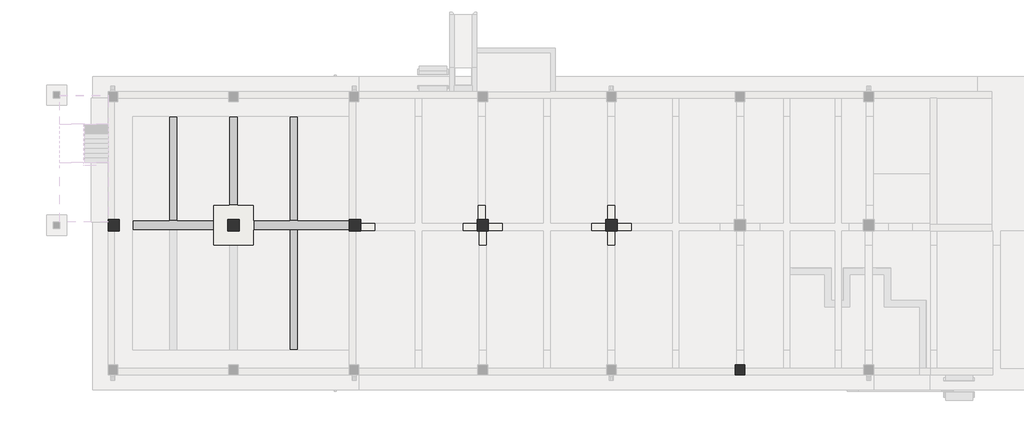
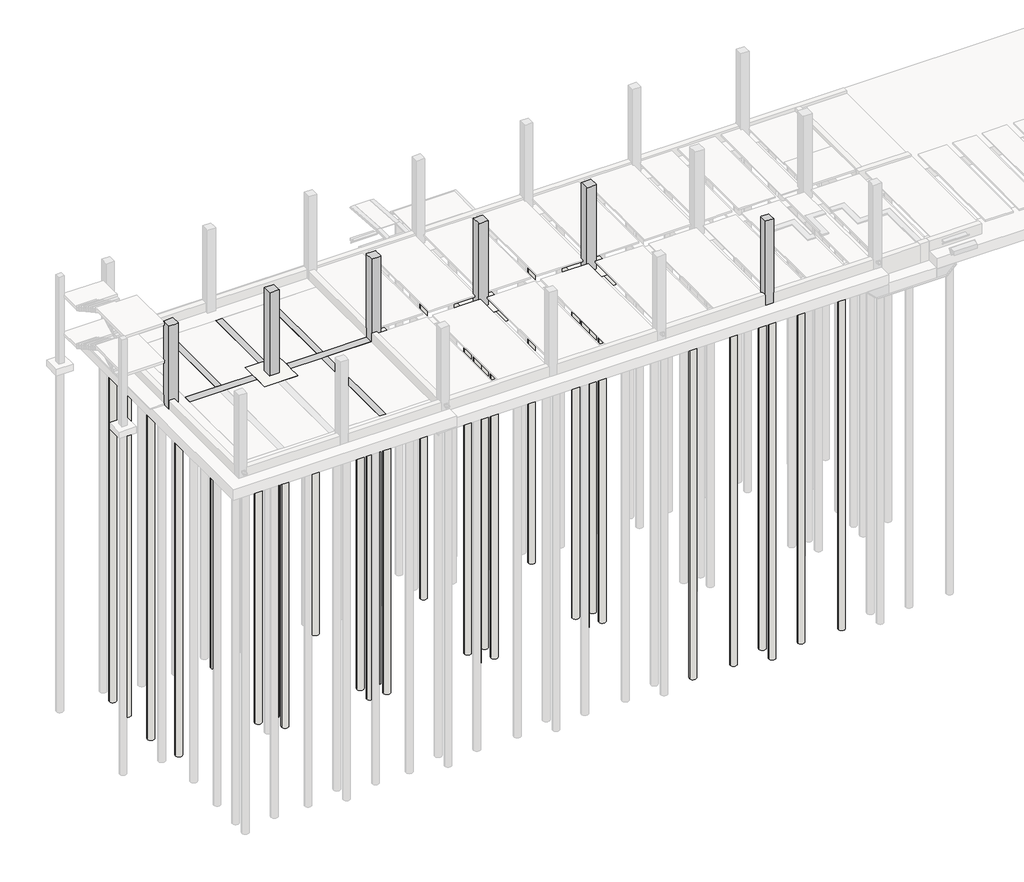
# One storey, part 4 of 7: 33 slabs, 8 beams, 6 columns.
"""IFC4 building model written with IfcOpenShell, lengths in millimetres."""

from ifc_helpers import new_model, si_unit, point, frame, frame_2d, origin, place, context, project, spatial, polyline, circle_curve, trimmed, segment, composite_curve, outline, extrude, faceted_brep, element, save

model = new_model("IFC4")

# Units and contexts
model_context = context("Model", 3, world=origin())
ifc_project = project(units=[si_unit("LENGTHUNIT", "METRE", prefix="MILLI")], contexts=[model_context])

# Site, building, storey
site = spatial("IfcSite", under=ifc_project)
building = spatial("IfcBuilding", under=site)
storey = spatial("IfcBuildingStorey", under=building, Name="H.P.P", Elevation=4500.0)

# Beams
placement = place(None, origin())
element("IfcBeam", 1, ObjectType="RC Beam_Rectangular : H_SB_AR S16_TG-UG_500x700_FB1A", at=placement, inside=storey, context=model_context, shape_type="Brep", body=[
    faceted_brep([(11000.0, -15750.0, 3400.0), (11500.0, -15750.0, 3400.0), (11500.0, -15750.0, 3840.0), (11500.0, -15750.0, 3950.0), (11500.0, -15750.0, 4100.0), (11000.0, -15750.0, 4100.0), (11000.0, -15750.0, 3950.0), (11000.0, -15750.0, 3840.0), (11500.0, -8299.9999999, 4100.0), (11000.0, -8299.9999999, 4100.0), (11500.0, -8299.9999999, 3950.0), (11500.0, -8299.9999999, 3400.0), (11500.0, -8299.9999999, 3840.0), (11000.0, -8299.9999999, 3400.0), (11000.0, -8299.9999999, 3950.0), (11000.0, -8299.9999999, 3840.0)], [[[0, 1, 2, 3, 4, 5, 6, 7]], [[5, 4, 8, 9]], [[10, 8, 4, 3, 2, 1, 11, 12]], [[1, 0, 13, 11]], [[9, 14, 15, 13, 0, 7, 6, 5]], [[9, 8, 10, 12, 11, 13, 15, 14]]]),
])
element("IfcBeam", 2, ObjectType="RC Beam_Rectangular : H_SB_AR S16_TG-UG_600x800_FG2", at=placement, inside=storey, context=model_context, shape_type="Brep", body=[
    faceted_brep([(6250.0000003, -7700.0, 4100.0), (6250.0000003, -8300.0, 4100.0), (6250.0000003, -8300.0, 3950.0), (6250.0000003, -8300.0, 3840.0), (6250.0000003, -8300.0, 3300.0), (6250.0000003, -7700.0, 3300.0), (6250.0000003, -7700.0, 3840.0), (6250.0000003, -7700.0, 3950.0), (1250.0000003, -7700.0, 3300.0), (1250.0000003, -8300.0, 3300.0), (1250.0000003, -8300.0, 3840.0), (1250.0000003, -8300.0, 3950.0), (1250.0000003, -8300.0, 4100.0), (1250.0000003, -7700.0, 4100.0), (1250.0000003, -7700.0, 3950.0), (1250.0000003, -7700.0, 3840.0), (4000.0, -7700.0, 4100.0), (3500.0, -7700.0, 4100.0), (3500.0, -8300.0, 4100.0), (4000.0, -8300.0, 4100.0)], [[[0, 1, 2, 3, 4, 5, 6, 7]], [[8, 9, 10, 11, 12, 13, 14, 15]], [[1, 0, 16, 17, 13, 12, 18, 19]], [[9, 4, 3, 2, 1, 19, 18, 12, 11, 10]], [[5, 4, 9, 8]], [[5, 8, 15, 14, 13, 17, 16, 0, 7, 6]]]),
])
element("IfcBeam", 3, ObjectType="RC Beam_Rectangular : H_SB_AR S16_TG-UG_600x800_FG2", at=placement, inside=storey, context=model_context, shape_type="Brep", body=[
    faceted_brep([(8750.0000003, -7699.9999999, 3300.0), (8750.0000003, -8299.9999999, 3300.0), (8750.0000003, -8299.9999999, 3840.0), (8750.0000003, -8299.9999999, 3950.0), (8750.0000003, -8299.9999999, 4100.0), (8750.0000003, -7699.9999999, 4100.0), (8750.0000003, -7699.9999999, 3950.0), (8750.0000003, -7699.9999999, 3840.0), (11000.0, -8299.9999999, 4100.0), (11500.0, -8299.9999999, 4100.0), (14700.0000001, -8299.9999999, 4100.0), (14700.0000001, -7699.9999999, 4100.0), (11500.0, -7699.9999999, 4100.0), (11000.0, -7699.9999999, 4100.0), (13800.0000001, -8299.9999999, 4000.0), (14700.0000001, -8299.9999999, 4000.0), (13800.0000001, -8299.9999999, 3300.0), (13800.0000001, -8299.9999999, 3840.0), (13800.0000001, -8299.9999999, 3950.0), (13800.0000001, -7699.9999999, 3300.0), (14700.0000001, -7699.9999999, 4000.0), (13800.0000001, -7699.9999999, 4000.0), (13800.0000001, -7699.9999999, 3950.0), (13800.0000001, -7699.9999999, 3840.0)], [[[0, 1, 2, 3, 4, 5, 6, 7]], [[5, 4, 8, 9, 10, 11, 12, 13]], [[14, 15, 10, 9, 8, 4, 3, 2, 1, 16, 17, 18]], [[1, 0, 19, 16]], [[20, 21, 22, 23, 19, 0, 7, 6, 5, 13, 12, 11]], [[14, 21, 20, 15]], [[21, 14, 18, 17, 16, 19, 23, 22]], [[11, 10, 15, 20]]]),
])
element("IfcBeam", 4, ObjectType="RC Beam_Rectangular : H_SB_AR S16_TG-UG_500x700_FG1", at=placement, inside=storey, context=model_context, shape_type="Brep", body=[
    faceted_brep([(14700.0249709, -15746.4519217, 4100.0), (14700.0249709, -15746.4519217, 3400.0), (14975.0010428, -15750.0000001, 3400.0), (14975.0010428, -15750.0000001, 4100.0), (15200.0208108, -15750.0000001, 4100.0), (15295.5046819, -8350.0, 4100.0), (15100.0, -8350.0, 4100.0), (14795.4630603, -8350.0, 4100.0), (15200.0208108, -15750.0000001, 3400.0), (15283.8917786, -9250.0, 3400.0), (15283.8917786, -9250.0, 4000.0), (15295.5046819, -8350.0, 4000.0), (14783.8501571, -9250.0, 3400.0), (14795.4630603, -8350.0, 4000.0), (14783.8501571, -9250.0, 4000.0)], [[[0, 1, 2, 3]], [[3, 4, 5, 6, 7, 0]], [[4, 8, 9, 10, 11, 5]], [[8, 2, 1, 12, 9]], [[1, 0, 7, 13, 14, 12]], [[4, 3, 2, 8]], [[10, 14, 13, 11]], [[10, 9, 12, 14]], [[7, 6, 5, 11, 13]]]),
])
element("IfcBeam", 5, ObjectType="RC Beam_Rectangular : H_SB_AR S16_TG-UG_500x700_FB1A", at=placement, inside=storey, context=model_context, shape_type="Brep", body=[
    faceted_brep([(4000.0, -1250.0000001, 3400.0), (3500.0, -1250.0000001, 3400.0), (3500.0, -1250.0000001, 3840.0), (3500.0, -1250.0000001, 3950.0), (3500.0, -1250.0000001, 4100.0), (4000.0, -1250.0000001, 4100.0), (4000.0, -1250.0000001, 3950.0), (4000.0, -1250.0000001, 3840.0), (3500.0, -7700.0, 4100.0), (4000.0, -7700.0, 4100.0), (4000.0, -7700.0, 3950.0), (4000.0, -7700.0, 3840.0), (4000.0, -7700.0, 3400.0), (3500.0, -7700.0, 3400.0), (3500.0, -7700.0, 3840.0), (3500.0, -7700.0, 3950.0)], [[[0, 1, 2, 3, 4, 5, 6, 7]], [[5, 4, 8, 9]], [[5, 9, 10, 11, 12, 0, 7, 6]], [[1, 0, 12, 13]], [[8, 4, 3, 2, 1, 13, 14, 15]], [[9, 8, 15, 14, 13, 12, 11, 10]]]),
])
element("IfcBeam", 6, ObjectType="RC Beam_Rectangular : H_SB_AR S16_TG-UG_500x700_FG1", at=placement, inside=storey, context=model_context, shape_type="Brep", body=[
    faceted_brep([(7750.0, -6750.0000001, 4100.0), (7250.0, -6750.0000001, 4100.0), (7250.0, -6750.0000001, 3950.0), (7250.0, -6750.0000001, 3840.0), (7250.0, -6750.0000001, 3400.0), (7750.0, -6750.0000001, 3400.0), (7750.0, -6750.0000001, 3840.0), (7750.0, -6750.0000001, 3950.0), (7750.0, -1250.0000001, 3400.0), (7250.0, -1250.0000001, 3400.0), (7250.0, -1250.0000001, 3840.0), (7250.0, -1250.0000001, 3950.0), (7250.0, -1250.0000001, 4100.0), (7750.0, -1250.0000001, 4100.0), (7750.0, -1250.0000001, 3950.0), (7750.0, -1250.0000001, 3840.0)], [[[0, 1, 2, 3, 4, 5, 6, 7]], [[8, 9, 10, 11, 12, 13, 14, 15]], [[1, 0, 13, 12]], [[13, 0, 7, 6, 5, 8, 15, 14]], [[5, 4, 9, 8]], [[1, 12, 11, 10, 9, 4, 3, 2]]]),
])
element("IfcBeam", 7, ObjectType="RC Beam_Rectangular : H_SB_AR S16_TG-UG_500x700_FB1A", at=placement, inside=storey, context=model_context, shape_type="Brep", body=[
    faceted_brep([(11500.0, -1250.0000001, 3400.0), (11000.0, -1250.0000001, 3400.0), (11000.0, -1250.0000001, 3840.0), (11000.0, -1250.0000001, 3950.0), (11000.0, -1250.0000001, 4100.0), (11500.0, -1250.0000001, 4100.0), (11500.0, -1250.0000001, 3950.0), (11500.0, -1250.0000001, 3840.0), (11000.0, -7699.9999999, 4100.0), (11500.0, -7699.9999999, 4100.0), (11500.0, -7699.9999999, 3950.0), (11500.0, -7699.9999999, 3840.0), (11500.0, -7699.9999999, 3400.0), (11000.0, -7699.9999999, 3400.0), (11000.0, -7699.9999999, 3840.0), (11000.0, -7699.9999999, 3950.0)], [[[0, 1, 2, 3, 4, 5, 6, 7]], [[5, 4, 8, 9]], [[5, 9, 10, 11, 12, 0, 7, 6]], [[1, 0, 12, 13]], [[8, 4, 3, 2, 1, 13, 14, 15]], [[9, 8, 15, 14, 13, 12, 11, 10]]]),
])
element("IfcBeam", 8, ObjectType="RC Beam_Rectangular : H_SB_AR S16_TG-UG_500x700_FG1", at=placement, inside=storey, context=model_context, shape_type="Brep", body=[
    faceted_brep([(14700.0329164, -1254.0736068, 3400.0), (14700.0329164, -1254.0736068, 4100.0), (14975.0013677, -1250.0000001, 4100.0), (14975.0013677, -1250.0000001, 3400.0), (15200.0274333, -1250.0000001, 4100.0), (14794.7873816, -7650.0, 4100.0), (15100.0, -7650.0, 4100.0), (15294.8422483, -7650.0, 4100.0), (15200.0274333, -1250.0000001, 3400.0), (15294.8422483, -7650.0, 4000.0), (15281.5089149, -6750.0, 4000.0), (15281.5089149, -6750.0, 3400.0), (14781.4540482, -6750.0, 3400.0), (14781.4540482, -6750.0, 4000.0), (14794.7873816, -7650.0, 4000.0)], [[[0, 1, 2, 3]], [[4, 2, 1, 5, 6, 7]], [[8, 4, 7, 9, 10, 11]], [[3, 8, 11, 12, 0]], [[1, 0, 12, 13, 14, 5]], [[2, 4, 8, 3]], [[13, 10, 9, 14]], [[10, 13, 12, 11]], [[7, 6, 5, 14, 9]]]),
])

# Columns
element("IfcColumn", 9, ObjectType="RC_Column_Rectangular : H_SC_AR S15_RC Col-AG_700x700_C1", at=placement, inside=storey, context=model_context, shape_type="Brep", body=[
    faceted_brep([(400.0, -7650.0, 4100.0), (400.0, -8350.0, 4100.0), (100.0, -8350.0, 4100.0), (-300.0, -8350.0, 4100.0), (-300.0, -7650.0, 4100.0), (100.0, -7650.0, 4100.0), (400.0, -7650.0, 10450.0), (400.0, -7700.0, 10450.0), (400.0, -7700.0, 10600.0), (400.0, -8300.0, 10600.0), (400.0, -8300.0, 10450.0), (400.0, -8350.0, 10450.0), (399.4974747, -8350.0, 10450.0), (399.4974747, -8350.0, 10600.0), (100.0, -8350.0, 10600.0), (-300.0, -8350.0, 10600.0), (-300.0, -8350.0, 9900.0), (-300.0, -8350.0, 4800.0), (-300.0, -7650.0, 10600.0), (-300.0, -7650.0, 9900.0), (-300.0, -7650.0, 4800.0), (100.0, -7650.0, 10600.0), (399.4974747, -7650.0, 10600.0), (399.4974747, -7650.0, 10450.0), (399.4974747, -8300.0, 10600.0), (399.4974747, -7700.0, 10600.0), (399.4974747, -7700.0, 10450.0), (399.4974747, -8300.0, 10450.0)], [[[0, 1, 2, 3, 4, 5]], [[1, 0, 6, 7, 8, 9, 10, 11]], [[3, 2, 1, 11, 12, 13, 14, 15, 16, 17]], [[4, 3, 17, 16, 15, 18, 19, 20]], [[0, 5, 4, 20, 19, 18, 21, 22, 23, 6]], [[18, 15, 14, 13, 24, 9, 8, 25, 22, 21]], [[23, 26, 7, 6]], [[26, 25, 8, 7]], [[26, 23, 22, 25]], [[12, 27, 24, 13]], [[24, 27, 10, 9]], [[27, 12, 11, 10]]]),
])
element("IfcColumn", 10, ObjectType="RC_Column_Rectangular : H_SC_AR S15_RC Col-AG_700x700_C1", at=placement, inside=storey, context=model_context, shape_type="Brep", body=[
    faceted_brep([(7850.0, -7650.0, 4100.0), (7850.0, -8350.0, 4100.0), (7150.0, -8350.0, 4100.0), (7150.0, -7650.0, 4100.0), (7850.0, -7650.0, 10450.0), (7850.0, -7650.0, 10600.0), (7850.0, -7700.0, 10600.0), (7850.0, -8300.0, 10600.0), (7850.0, -8350.0, 10600.0), (7850.0, -8350.0, 10450.0), (7750.0, -8350.0, 10600.0), (7250.0, -8350.0, 10600.0), (7150.0, -8350.0, 10600.0), (7150.0, -8350.0, 10450.0), (7150.0, -8300.0, 10600.0), (7150.0, -7700.0, 10600.0), (7150.0, -7650.0, 10600.0), (7150.0, -7650.0, 10450.0), (7250.0, -7650.0, 10600.0), (7750.0, -7650.0, 10600.0)], [[[0, 1, 2, 3]], [[1, 0, 4, 5, 6, 7, 8, 9]], [[2, 1, 9, 8, 10, 11, 12, 13]], [[3, 2, 13, 12, 14, 15, 16, 17]], [[0, 3, 17, 16, 18, 19, 5, 4]], [[18, 16, 15, 14, 12, 11, 10, 8, 7, 6, 5, 19]]]),
])
element("IfcColumn", 11, ObjectType="RC_Column_Rectangular : H_SC_AR S15_RC Col-AG_700x700_C1", at=placement, inside=storey, context=model_context, shape_type="Brep", body=[
    faceted_brep([(15400.0000001, -7650.0, 4000.0), (15400.0000001, -7850.0, 4000.0), (15400.0000001, -8350.0, 4000.0), (15295.5046819, -8350.0, 4000.0), (14795.4630603, -8350.0, 4000.0), (14700.0000001, -8350.0, 4000.0), (14700.0000001, -8299.9999999, 4000.0), (14700.0000001, -7699.9999999, 4000.0), (14700.0000001, -7650.0, 4000.0), (14794.7873816, -7650.0, 4000.0), (15294.8422483, -7650.0, 4000.0), (15400.0000001, -7650.0, 4650.0), (15400.0000001, -7650.0, 4800.0), (15400.0000001, -7650.0, 10450.0), (15400.0000001, -7650.0, 10600.0), (15400.0000001, -7700.0, 10600.0), (15400.0000001, -8300.0, 10600.0), (15400.0000001, -8350.0, 10600.0), (15400.0000001, -8350.0, 10450.0), (15400.0000001, -8350.0, 4800.0), (15400.0000001, -8350.0, 4650.0), (15200.0, -8350.0, 10600.0), (14700.0000001, -8350.0, 10600.0), (14700.0000001, -8350.0, 10450.0), (14700.0000001, -8350.0, 4800.0), (14700.0000001, -8350.0, 4100.0), (14700.0000001, -8300.0, 10600.0), (14700.0000001, -7700.0, 10600.0), (14700.0000001, -7650.0, 10600.0), (14700.0000001, -7650.0, 10450.0), (14700.0000001, -7650.0, 4800.0), (14700.0000001, -7650.0, 4100.0), (15200.0, -7650.0, 10600.0)], [[[0, 1, 2, 3, 4, 5, 6, 7, 8, 9, 10]], [[2, 1, 0, 11, 12, 13, 14, 15, 16, 17, 18, 19, 20]], [[5, 4, 3, 2, 20, 19, 18, 17, 21, 22, 23, 24, 25]], [[8, 7, 6, 5, 25, 24, 23, 22, 26, 27, 28, 29, 30, 31]], [[0, 10, 9, 8, 31, 30, 29, 28, 32, 14, 13, 12, 11]], [[15, 14, 32, 28, 27, 26, 22, 21, 17, 16]]]),
])
element("IfcColumn", 12, ObjectType="RC_Column_Rectangular : H_SC_AR S15_RC Col-AG_700x700_C1", at=placement, inside=storey, context=model_context, shape_type="Brep", body=[
    faceted_brep([(23350.0000003, -7650.0, 4000.0), (23350.0000003, -8350.0, 4000.0), (23250.0, -8350.0, 4000.0), (22750.0, -8350.0, 4000.0), (22650.0000003, -8350.0, 4000.0), (22650.0000003, -7650.0, 4000.0), (22700.0, -7650.0, 4000.0), (23200.0, -7650.0, 4000.0), (23350.0000003, -7650.0, 4650.0), (23350.0000003, -7650.0, 4800.0), (23350.0000003, -7650.0, 10450.0), (23350.0000003, -7650.0, 10600.0), (23350.0000003, -7700.0, 10600.0), (23350.0000003, -8300.0, 10600.0), (23350.0000003, -8350.0, 10600.0), (23350.0000003, -8350.0, 10450.0), (23350.0000003, -8350.0, 4800.0), (23350.0000003, -8350.0, 4650.0), (23200.0, -8350.0, 10600.0), (22700.0, -8350.0, 10600.0), (22650.0000003, -8350.0, 10600.0), (22650.0000003, -8350.0, 10450.0), (22650.0000003, -8350.0, 4800.0), (22650.0000003, -8350.0, 4650.0), (22650.0000003, -8300.0, 10600.0), (22650.0000003, -7700.0, 10600.0), (22650.0000003, -7650.0, 10600.0), (22650.0000003, -7650.0, 10450.0), (22650.0000003, -7650.0, 4800.0), (22650.0000003, -7650.0, 4650.0), (22700.0, -7650.0, 10600.0), (23200.0, -7650.0, 10600.0)], [[[0, 1, 2, 3, 4, 5, 6, 7]], [[1, 0, 8, 9, 10, 11, 12, 13, 14, 15, 16, 17]], [[4, 3, 2, 1, 17, 16, 15, 14, 18, 19, 20, 21, 22, 23]], [[5, 4, 23, 22, 21, 20, 24, 25, 26, 27, 28, 29]], [[0, 7, 6, 5, 29, 28, 27, 26, 30, 31, 11, 10, 9, 8]], [[12, 11, 31, 30, 26, 25, 24, 20, 19, 18, 14, 13]]]),
])
element("IfcColumn", 13, ObjectType="RC_Column_Rectangular : H_SC_AR S15_RC Col-AG_700x700_C1", at=placement, inside=storey, context=model_context, shape_type="Brep", body=[
    faceted_brep([(31350.0000002, -7650.0, 4000.0), (31350.0000002, -8350.0, 4000.0), (31250.0, -8350.0, 4000.0), (30750.0, -8350.0, 4000.0), (30650.0000002, -8350.0, 4000.0), (30650.0000002, -7650.0, 4000.0), (30750.0, -7650.0, 4000.0), (31250.0, -7650.0, 4000.0), (31350.0000002, -7650.0, 4650.0), (31350.0000002, -7650.0, 4800.0), (31350.0000002, -7650.0, 10450.0), (31350.0000002, -7650.0, 10600.0), (31350.0000002, -7700.0, 10600.0), (31350.0000002, -8300.0, 10600.0), (31350.0000002, -8350.0, 10600.0), (31350.0000002, -8350.0, 10450.0), (31350.0000002, -8350.0, 4800.0), (31350.0000002, -8350.0, 4650.0), (31249.9999998, -8350.0, 10600.0), (30750.0000002, -8350.0, 10600.0), (30650.0000002, -8350.0, 10600.0), (30650.0000002, -8350.0, 10450.0), (30650.0000002, -8350.0, 4800.0), (30650.0000002, -8350.0, 4650.0), (30650.0000002, -8300.0, 10600.0), (30650.0000002, -7700.0, 10600.0), (30650.0000002, -7650.0, 10600.0), (30650.0000002, -7650.0, 10450.0), (30650.0000002, -7650.0, 4800.0), (30650.0000002, -7650.0, 4650.0), (30750.0000002, -7650.0, 10600.0), (31249.9999998, -7650.0, 10600.0)], [[[0, 1, 2, 3, 4, 5, 6, 7]], [[1, 0, 8, 9, 10, 11, 12, 13, 14, 15, 16, 17]], [[4, 3, 2, 1, 17, 16, 15, 14, 18, 19, 20, 21, 22, 23]], [[5, 4, 23, 22, 21, 20, 24, 25, 26, 27, 28, 29]], [[0, 7, 6, 5, 29, 28, 27, 26, 30, 31, 11, 10, 9, 8]], [[12, 11, 31, 30, 26, 25, 24, 20, 19, 18, 14, 13]]]),
])
element("IfcColumn", 14, ObjectType="RC_Column_Rectangular : H_SC_AR S15_RC Col-AG_600x600_C2", at=placement, inside=storey, context=model_context, shape_type="Brep", body=[
    faceted_brep([(38700.0, -16700.0, 4000.0), (39300.0, -16700.0, 4000.0), (39300.0, -16900.0, 4000.0), (39300.0, -17300.0, 4000.0), (38700.0, -17300.0, 4000.0), (38700.0, -16900.0, 4000.0), (38700.0, -16700.0, 4650.0), (38700.0, -16700.0, 4800.0), (38700.0, -16700.0, 10450.0), (38700.0, -16700.0, 10600.0), (38750.0000002, -16700.0, 10600.0), (39249.9999998, -16700.0, 10600.0), (39300.0, -16700.0, 10600.0), (39300.0, -16700.0, 10450.0), (39300.0, -16700.0, 4800.0), (39300.0, -16700.0, 4650.0), (39300.0, -16900.0, 10600.0), (39300.0, -17300.0, 10600.0), (39300.0, -17300.0, 9800.0), (39300.0, -17300.0, 4800.0), (38700.0, -17300.0, 10600.0), (38700.0, -17300.0, 9800.0), (38700.0, -17300.0, 4800.0), (38700.0, -16900.0, 10600.0)], [[[0, 1, 2, 3, 4, 5]], [[1, 0, 6, 7, 8, 9, 10, 11, 12, 13, 14, 15]], [[3, 2, 1, 15, 14, 13, 12, 16, 17, 18, 19]], [[4, 3, 19, 18, 17, 20, 21, 22]], [[0, 5, 4, 22, 21, 20, 23, 9, 8, 7, 6]], [[20, 17, 16, 12, 11, 10, 9, 23]]]),
])

# Slabs
element("IfcSlab", 15, ObjectType="Foundation Rectangular (Non-Pile) : H_SF_AR S18_Ret Fdn_2500x2500xT1000_F1", at=placement, inside=storey, context=model_context, shape_type="Brep", body=[
    faceted_brep([(8750.0, -6750.0, 4100.0), (7750.0, -6750.0, 4100.0), (7250.0, -6750.0, 4100.0), (6250.0, -6750.0, 4100.0), (6250.0, -7700.0, 4100.0), (6250.0, -8300.0, 4100.0), (6250.0, -9250.0, 4100.0), (7250.0, -9250.0, 4100.0), (7750.0, -9250.0, 4100.0), (8750.0, -9250.0, 4100.0), (8750.0, -8299.9999999, 4100.0), (8750.0, -7699.9999999, 4100.0), (8750.0, -6750.0, 3100.0), (8750.0, -9250.0, 3100.0), (6250.0, -9250.0, 3100.0), (6250.0, -6750.0, 3100.0), (8750.0, -6750.0, 3840.0), (8750.0, -6750.0, 3790.0), (6250.0, -6750.0, 3790.0), (6250.0, -6750.0, 3840.0), (6250.0, -9250.0, 3790.0), (6250.0, -9250.0, 3840.0), (8750.0, -9250.0, 3790.0), (8750.0, -9250.0, 3840.0)], [[[0, 1, 2, 3, 4, 5, 6, 7, 8, 9, 10, 11]], [[12, 13, 14, 15]], [[3, 2, 1, 0, 16, 17, 12, 15, 18, 19]], [[6, 5, 4, 3, 19, 18, 15, 14, 20, 21]], [[9, 8, 7, 6, 21, 20, 14, 13, 22, 23]], [[0, 11, 10, 9, 23, 22, 13, 12, 17, 16]]]),
])
element("IfcSlab", 16, ObjectType="Foundation Rectangular (Non-Pile) : H_SF_AR S18_Ret Fdn_2500x2500xT1000_F1A", at=placement, inside=storey, context=model_context, shape_type="Brep", body=[
    faceted_brep([(16300.0000001, -6750.0, 4000.0), (15281.5089149, -6750.0, 4000.0), (14781.4540482, -6750.0, 4000.0), (14700.0000001, -6750.0, 4000.0), (13800.0000001, -6750.0, 4000.0), (13800.0000001, -7699.9999999, 4000.0), (13800.0000001, -8299.9999999, 4000.0), (13800.0000001, -9250.0, 4000.0), (14700.0, -9250.0, 4000.0), (14783.8501571, -9250.0, 4000.0), (15283.8917786, -9250.0, 4000.0), (16300.0000001, -9250.0, 4000.0), (16300.0000001, -6750.0, 3000.0), (16300.0000001, -9250.0, 3000.0), (13800.0000001, -9250.0, 3000.0), (13800.0000001, -6750.0, 3000.0), (13800.0000001, -6750.0, 3790.0), (13800.0000001, -6750.0, 3840.0), (13800.0000001, -6750.0, 3950.0), (13800.0000001, -9250.0, 3790.0), (13800.0000001, -9250.0, 3840.0), (13800.0000001, -9250.0, 3950.0)], [[[0, 1, 2, 3, 4, 5, 6, 7, 8, 9, 10, 11]], [[12, 13, 14, 15]], [[4, 3, 2, 1, 0, 12, 15, 16, 17, 18]], [[7, 6, 5, 4, 18, 17, 16, 15, 14, 19, 20, 21]], [[11, 10, 9, 8, 7, 21, 20, 19, 14, 13]], [[0, 11, 13, 12]]]),
])
element("IfcSlab", 17, ObjectType="Foundation Rectangular (Non-Pile) : H_SF_AR S18_Ret Fdn_2500x2500xT1000_F1A", at=placement, inside=storey, context=model_context, shape_type="SweptSolid", body=[
    extrude(outline(polyline([(24250.0000003, -6750.0), (24250.0000003, -9250.0), (21750.0000003, -9250.0), (21750.0000003, -6750.0), (24250.0000003, -6750.0)])), frame((0.0, 0.0, 3000.0), z_axis=(0.0, 0.0, 1.0), x_axis=(1.0, 0.0, 0.0)), (0.0, 0.0, 1.0), 1000.0),
])
element("IfcSlab", 18, ObjectType="Foundation Rectangular (Non-Pile) : H_SF_AR S18_Ret Fdn_2500x2500xT1000_F1A", at=placement, inside=storey, context=model_context, shape_type="SweptSolid", body=[
    extrude(outline(polyline([(32250.0000002, -6750.0), (32250.0000002, -9250.0), (29750.0000002, -9250.0), (29750.0000002, -6750.0), (32250.0000002, -6750.0)])), frame((0.0, 0.0, 3000.0), z_axis=(0.0, 0.0, 1.0), x_axis=(1.0, 0.0, 0.0)), (0.0, 0.0, 1.0), 1000.0),
])
element("IfcSlab", 19, ObjectType="PILE : H_FL_AR S19_Pile_D500_L26.9", at=placement, inside=storey, context=model_context, shape_type="SweptSolid", body=[
    extrude(outline(composite_curve([segment(trimmed(circle_curve(frame_2d((0.0, -625.0000002)), 250.0), [point((-250.0, -625.0000002))], [point((250.0, -625.0000002))], False, "CARTESIAN"), True, "CONTINUOUS"), segment(trimmed(circle_curve(frame_2d((0.0, -625.0000002)), 250.0), [point((250.0, -625.0000002))], [point((-250.0, -625.0000002))], False, "CARTESIAN"), True, "CONTINUOUS")], self_intersect=False)), frame((0.0, 0.0, -23500.0), z_axis=(0.0, 0.0, 1.0), x_axis=(1.0, 0.0, 0.0)), (0.0, 0.0, 1.0), 26750.0),
])
element("IfcSlab", 20, ObjectType="PILE : H_FL_AR S19_Pile_D500_L26.9", at=placement, inside=storey, context=model_context, shape_type="SweptSolid", body=[
    extrude(outline(composite_curve([segment(trimmed(circle_curve(frame_2d((0.0, -2500.0000003)), 250.0), [point((-250.0, -2500.0000003))], [point((250.0, -2500.0000003))], False, "CARTESIAN"), True, "CONTINUOUS"), segment(trimmed(circle_curve(frame_2d((0.0, -2500.0000003)), 250.0), [point((250.0, -2500.0000003))], [point((-250.0, -2500.0000003))], False, "CARTESIAN"), True, "CONTINUOUS")], self_intersect=False)), frame((0.0, 0.0, -23500.0), z_axis=(0.0, 0.0, 1.0), x_axis=(1.0, 0.0, 0.0)), (0.0, 0.0, 1.0), 26750.0),
])
element("IfcSlab", 21, ObjectType="PILE : H_FL_AR S19_Pile_D500_L26.9", at=placement, inside=storey, context=model_context, shape_type="SweptSolid", body=[
    extrude(outline(composite_curve([segment(trimmed(circle_curve(frame_2d((0.0, -5500.0000003)), 250.0), [point((-250.0, -5500.0000003))], [point((250.0, -5500.0000003))], False, "CARTESIAN"), True, "CONTINUOUS"), segment(trimmed(circle_curve(frame_2d((0.0, -5500.0000003)), 250.0), [point((250.0, -5500.0000003))], [point((-250.0, -5500.0000003))], False, "CARTESIAN"), True, "CONTINUOUS")], self_intersect=False)), frame((0.0, 0.0, -23500.0), z_axis=(0.0, 0.0, 1.0), x_axis=(1.0, 0.0, 0.0)), (0.0, 0.0, 1.0), 26750.0),
])
element("IfcSlab", 22, ObjectType="PILE : H_FL_AR S19_Pile_D500_L26.9", at=placement, inside=storey, context=model_context, shape_type="SweptSolid", body=[
    extrude(outline(composite_curve([segment(trimmed(circle_curve(frame_2d((624.9999999, -8000.0)), 250.0), [point((374.9999999, -8000.0))], [point((874.9999999, -8000.0))], False, "CARTESIAN"), True, "CONTINUOUS"), segment(trimmed(circle_curve(frame_2d((624.9999999, -8000.0)), 250.0), [point((874.9999999, -8000.0))], [point((374.9999999, -8000.0))], False, "CARTESIAN"), True, "CONTINUOUS")], self_intersect=False)), frame((0.0, 0.0, -23500.0), z_axis=(0.0, 0.0, 1.0), x_axis=(1.0, 0.0, 0.0)), (0.0, 0.0, 1.0), 26750.0),
])
element("IfcSlab", 23, ObjectType="PILE : H_FL_AR S19_Pile_D500_L26.9", at=placement, inside=storey, context=model_context, shape_type="SweptSolid", body=[
    extrude(outline(composite_curve([segment(trimmed(circle_curve(frame_2d((7500.0, -625.0000001)), 250.0), [point((7250.0, -625.0000001))], [point((7750.0, -625.0000001))], False, "CARTESIAN"), True, "CONTINUOUS"), segment(trimmed(circle_curve(frame_2d((7500.0, -625.0000001)), 250.0), [point((7750.0, -625.0000001))], [point((7250.0, -625.0000001))], False, "CARTESIAN"), True, "CONTINUOUS")], self_intersect=False)), frame((0.0, 0.0, -23500.0), z_axis=(0.0, 0.0, 1.0), x_axis=(1.0, 0.0, 0.0)), (0.0, 0.0, 1.0), 26750.0),
])
element("IfcSlab", 24, ObjectType="PILE : H_FL_AR S19_Pile_D500_L26.8", at=placement, inside=storey, context=model_context, shape_type="SweptSolid", body=[
    extrude(outline(composite_curve([segment(trimmed(circle_curve(frame_2d((14999.9999999, -625.0000002)), 250.0), [point((15249.9999999, -625.0000002))], [point((14749.9999999, -625.0000002))], False, "CARTESIAN"), True, "CONTINUOUS"), segment(trimmed(circle_curve(frame_2d((14999.9999999, -625.0000002)), 250.0), [point((14749.9999999, -625.0000002))], [point((15249.9999999, -625.0000002))], False, "CARTESIAN"), True, "CONTINUOUS")], self_intersect=False)), frame((0.0, 0.0, 3200.0), z_axis=(0.0, 0.0, 1.0), x_axis=(1.0, 0.0, 0.0)), (0.0, 0.0, 1.0), 100.0),
    extrude(outline(composite_curve([segment(trimmed(circle_curve(frame_2d((14999.9999999, -625.0000002)), 250.0), [point((14749.9999999, -625.0000002))], [point((15249.9999999, -625.0000002))], False, "CARTESIAN"), True, "CONTINUOUS"), segment(trimmed(circle_curve(frame_2d((14999.9999999, -625.0000002)), 250.0), [point((15249.9999999, -625.0000002))], [point((14749.9999999, -625.0000002))], False, "CARTESIAN"), True, "CONTINUOUS")], self_intersect=False)), frame((0.0, 0.0, -23500.0), z_axis=(0.0, 0.0, 1.0), x_axis=(1.0, 0.0, 0.0)), (0.0, 0.0, 1.0), 26650.0),
])
element("IfcSlab", 25, ObjectType="PILE : H_FL_AR S19_Pile_D500_L26.8", at=placement, inside=storey, context=model_context, shape_type="SweptSolid", body=[
    extrude(outline(composite_curve([segment(trimmed(circle_curve(frame_2d((22999.9999996, -625.0000002)), 250.0), [point((22749.9999996, -625.0000002))], [point((23249.9999996, -625.0000002))], False, "CARTESIAN"), True, "CONTINUOUS"), segment(trimmed(circle_curve(frame_2d((22999.9999996, -625.0000002)), 250.0), [point((23249.9999996, -625.0000002))], [point((22749.9999996, -625.0000002))], False, "CARTESIAN"), True, "CONTINUOUS")], self_intersect=False)), frame((0.0, 0.0, -23500.0), z_axis=(0.0, 0.0, 1.0), x_axis=(1.0, 0.0, 0.0)), (0.0, 0.0, 1.0), 26650.0),
])
element("IfcSlab", 26, ObjectType="PILE : H_FL_AR S19_Pile_D500_L26.8", at=placement, inside=storey, context=model_context, shape_type="SweptSolid", body=[
    extrude(outline(composite_curve([segment(trimmed(circle_curve(frame_2d((31000.0, -625.0000001)), 250.0), [point((30750.0, -625.0000001))], [point((31250.0, -625.0000001))], False, "CARTESIAN"), True, "CONTINUOUS"), segment(trimmed(circle_curve(frame_2d((31000.0, -625.0000001)), 250.0), [point((31250.0, -625.0000001))], [point((30750.0, -625.0000001))], False, "CARTESIAN"), True, "CONTINUOUS")], self_intersect=False)), frame((0.0, 0.0, -23500.0), z_axis=(0.0, 0.0, 1.0), x_axis=(1.0, 0.0, 0.0)), (0.0, 0.0, 1.0), 26650.0),
])
element("IfcSlab", 27, ObjectType="PILE : H_FL_AR S19_Pile_D500_L26.7", at=placement, inside=storey, context=model_context, shape_type="SweptSolid", body=[
    extrude(outline(composite_curve([segment(trimmed(circle_curve(frame_2d((6875.0000004, -7374.9999999)), 250.0), [point((6625.0000004, -7374.9999999))], [point((7125.0000004, -7374.9999999))], False, "CARTESIAN"), True, "CONTINUOUS"), segment(trimmed(circle_curve(frame_2d((6875.0000004, -7374.9999999)), 250.0), [point((7125.0000004, -7374.9999999))], [point((6625.0000004, -7374.9999999))], False, "CARTESIAN"), True, "CONTINUOUS")], self_intersect=False)), frame((0.0, 0.0, -23500.0), z_axis=(0.0, 0.0, 1.0), x_axis=(1.0, 0.0, 0.0)), (0.0, 0.0, 1.0), 26550.0),
])
element("IfcSlab", 28, ObjectType="PILE : H_FL_AR S19_Pile_D500_L26.7", at=placement, inside=storey, context=model_context, shape_type="SweptSolid", body=[
    extrude(outline(composite_curve([segment(trimmed(circle_curve(frame_2d((8125.0000004, -7374.9999999)), 250.0), [point((7875.0000004, -7374.9999999))], [point((8375.0000004, -7374.9999999))], False, "CARTESIAN"), True, "CONTINUOUS"), segment(trimmed(circle_curve(frame_2d((8125.0000004, -7374.9999999)), 250.0), [point((8375.0000004, -7374.9999999))], [point((7875.0000004, -7374.9999999))], False, "CARTESIAN"), True, "CONTINUOUS")], self_intersect=False)), frame((0.0, 0.0, -23500.0), z_axis=(0.0, 0.0, 1.0), x_axis=(1.0, 0.0, 0.0)), (0.0, 0.0, 1.0), 26550.0),
])
element("IfcSlab", 29, ObjectType="PILE : H_FL_AR S19_Pile_D500_L26.7", at=placement, inside=storey, context=model_context, shape_type="SweptSolid", body=[
    extrude(outline(composite_curve([segment(trimmed(circle_curve(frame_2d((8125.0000004, -8624.9999999)), 250.0), [point((7875.0000004, -8624.9999999))], [point((8375.0000004, -8624.9999999))], False, "CARTESIAN"), True, "CONTINUOUS"), segment(trimmed(circle_curve(frame_2d((8125.0000004, -8624.9999999)), 250.0), [point((8375.0000004, -8624.9999999))], [point((7875.0000004, -8624.9999999))], False, "CARTESIAN"), True, "CONTINUOUS")], self_intersect=False)), frame((0.0, 0.0, -23500.0), z_axis=(0.0, 0.0, 1.0), x_axis=(1.0, 0.0, 0.0)), (0.0, 0.0, 1.0), 26550.0),
])
element("IfcSlab", 30, ObjectType="PILE : H_FL_AR S19_Pile_D500_L26.6", at=placement, inside=storey, context=model_context, shape_type="SweptSolid", body=[
    extrude(outline(composite_curve([segment(trimmed(circle_curve(frame_2d((14425.0000004, -7374.9999999)), 250.0), [point((14175.0000004, -7374.9999999))], [point((14675.0000004, -7374.9999999))], False, "CARTESIAN"), True, "CONTINUOUS"), segment(trimmed(circle_curve(frame_2d((14425.0000004, -7374.9999999)), 250.0), [point((14675.0000004, -7374.9999999))], [point((14175.0000004, -7374.9999999))], False, "CARTESIAN"), True, "CONTINUOUS")], self_intersect=False)), frame((0.0, 0.0, -23500.0), z_axis=(0.0, 0.0, 1.0), x_axis=(1.0, 0.0, 0.0)), (0.0, 0.0, 1.0), 26450.0),
])
element("IfcSlab", 31, ObjectType="PILE : H_FL_AR S19_Pile_D500_L26.6", at=placement, inside=storey, context=model_context, shape_type="SweptSolid", body=[
    extrude(outline(composite_curve([segment(trimmed(circle_curve(frame_2d((15675.0000004, -7374.9999999)), 250.0), [point((15425.0000004, -7374.9999999))], [point((15925.0000004, -7374.9999999))], False, "CARTESIAN"), True, "CONTINUOUS"), segment(trimmed(circle_curve(frame_2d((15675.0000004, -7374.9999999)), 250.0), [point((15925.0000004, -7374.9999999))], [point((15425.0000004, -7374.9999999))], False, "CARTESIAN"), True, "CONTINUOUS")], self_intersect=False)), frame((0.0, 0.0, -23500.0), z_axis=(0.0, 0.0, 1.0), x_axis=(1.0, 0.0, 0.0)), (0.0, 0.0, 1.0), 26450.0),
])
element("IfcSlab", 32, ObjectType="PILE : H_FL_AR S19_Pile_D500_L26.6", at=placement, inside=storey, context=model_context, shape_type="SweptSolid", body=[
    extrude(outline(composite_curve([segment(trimmed(circle_curve(frame_2d((14425.0000004, -8624.9999999)), 250.0), [point((14175.0000004, -8624.9999999))], [point((14675.0000004, -8624.9999999))], False, "CARTESIAN"), True, "CONTINUOUS"), segment(trimmed(circle_curve(frame_2d((14425.0000004, -8624.9999999)), 250.0), [point((14675.0000004, -8624.9999999))], [point((14175.0000004, -8624.9999999))], False, "CARTESIAN"), True, "CONTINUOUS")], self_intersect=False)), frame((0.0, 0.0, -23500.0), z_axis=(0.0, 0.0, 1.0), x_axis=(1.0, 0.0, 0.0)), (0.0, 0.0, 1.0), 26450.0),
])
element("IfcSlab", 33, ObjectType="PILE : H_FL_AR S19_Pile_D500_L26.6", at=placement, inside=storey, context=model_context, shape_type="SweptSolid", body=[
    extrude(outline(composite_curve([segment(trimmed(circle_curve(frame_2d((15675.0000004, -8624.9999999)), 250.0), [point((15425.0000004, -8624.9999999))], [point((15925.0000004, -8624.9999999))], False, "CARTESIAN"), True, "CONTINUOUS"), segment(trimmed(circle_curve(frame_2d((15675.0000004, -8624.9999999)), 250.0), [point((15925.0000004, -8624.9999999))], [point((15425.0000004, -8624.9999999))], False, "CARTESIAN"), True, "CONTINUOUS")], self_intersect=False)), frame((0.0, 0.0, -23500.0), z_axis=(0.0, 0.0, 1.0), x_axis=(1.0, 0.0, 0.0)), (0.0, 0.0, 1.0), 26450.0),
])
element("IfcSlab", 34, ObjectType="PILE : H_FL_AR S19_Pile_D500_L26.6", at=placement, inside=storey, context=model_context, shape_type="SweptSolid", body=[
    extrude(outline(composite_curve([segment(trimmed(circle_curve(frame_2d((22375.0000006, -7374.9999999)), 250.0), [point((22125.0000006, -7374.9999999))], [point((22625.0000006, -7374.9999999))], False, "CARTESIAN"), True, "CONTINUOUS"), segment(trimmed(circle_curve(frame_2d((22375.0000006, -7374.9999999)), 250.0), [point((22625.0000006, -7374.9999999))], [point((22125.0000006, -7374.9999999))], False, "CARTESIAN"), True, "CONTINUOUS")], self_intersect=False)), frame((0.0, 0.0, -23500.0), z_axis=(0.0, 0.0, 1.0), x_axis=(1.0, 0.0, 0.0)), (0.0, 0.0, 1.0), 26450.0),
])
element("IfcSlab", 35, ObjectType="PILE : H_FL_AR S19_Pile_D500_L26.6", at=placement, inside=storey, context=model_context, shape_type="SweptSolid", body=[
    extrude(outline(composite_curve([segment(trimmed(circle_curve(frame_2d((23625.0000006, -7374.9999999)), 250.0), [point((23375.0000006, -7374.9999999))], [point((23875.0000006, -7374.9999999))], False, "CARTESIAN"), True, "CONTINUOUS"), segment(trimmed(circle_curve(frame_2d((23625.0000006, -7374.9999999)), 250.0), [point((23875.0000006, -7374.9999999))], [point((23375.0000006, -7374.9999999))], False, "CARTESIAN"), True, "CONTINUOUS")], self_intersect=False)), frame((0.0, 0.0, -23500.0), z_axis=(0.0, 0.0, 1.0), x_axis=(1.0, 0.0, 0.0)), (0.0, 0.0, 1.0), 26450.0),
])
element("IfcSlab", 36, ObjectType="PILE : H_FL_AR S19_Pile_D500_L26.6", at=placement, inside=storey, context=model_context, shape_type="SweptSolid", body=[
    extrude(outline(composite_curve([segment(trimmed(circle_curve(frame_2d((22375.0000006, -8624.9999999)), 250.0), [point((22125.0000006, -8624.9999999))], [point((22625.0000006, -8624.9999999))], False, "CARTESIAN"), True, "CONTINUOUS"), segment(trimmed(circle_curve(frame_2d((22375.0000006, -8624.9999999)), 250.0), [point((22625.0000006, -8624.9999999))], [point((22125.0000006, -8624.9999999))], False, "CARTESIAN"), True, "CONTINUOUS")], self_intersect=False)), frame((0.0, 0.0, -23500.0), z_axis=(0.0, 0.0, 1.0), x_axis=(1.0, 0.0, 0.0)), (0.0, 0.0, 1.0), 26450.0),
])
element("IfcSlab", 37, ObjectType="PILE : H_FL_AR S19_Pile_D500_L26.6", at=placement, inside=storey, context=model_context, shape_type="SweptSolid", body=[
    extrude(outline(composite_curve([segment(trimmed(circle_curve(frame_2d((23625.0000006, -8624.9999999)), 250.0), [point((23375.0000006, -8624.9999999))], [point((23875.0000006, -8624.9999999))], False, "CARTESIAN"), True, "CONTINUOUS"), segment(trimmed(circle_curve(frame_2d((23625.0000006, -8624.9999999)), 250.0), [point((23875.0000006, -8624.9999999))], [point((23375.0000006, -8624.9999999))], False, "CARTESIAN"), True, "CONTINUOUS")], self_intersect=False)), frame((0.0, 0.0, -23500.0), z_axis=(0.0, 0.0, 1.0), x_axis=(1.0, 0.0, 0.0)), (0.0, 0.0, 1.0), 26450.0),
])
element("IfcSlab", 38, ObjectType="PILE : H_FL_AR S19_Pile_D500_L26.6", at=placement, inside=storey, context=model_context, shape_type="SweptSolid", body=[
    extrude(outline(composite_curve([segment(trimmed(circle_curve(frame_2d((30375.0000004, -7374.9999999)), 250.0), [point((30125.0000004, -7374.9999999))], [point((30625.0000004, -7374.9999999))], False, "CARTESIAN"), True, "CONTINUOUS"), segment(trimmed(circle_curve(frame_2d((30375.0000004, -7374.9999999)), 250.0), [point((30625.0000004, -7374.9999999))], [point((30125.0000004, -7374.9999999))], False, "CARTESIAN"), True, "CONTINUOUS")], self_intersect=False)), frame((0.0, 0.0, -23500.0), z_axis=(0.0, 0.0, 1.0), x_axis=(1.0, 0.0, 0.0)), (0.0, 0.0, 1.0), 26450.0),
])
element("IfcSlab", 39, ObjectType="PILE : H_FL_AR S19_Pile_D500_L26.6", at=placement, inside=storey, context=model_context, shape_type="SweptSolid", body=[
    extrude(outline(composite_curve([segment(trimmed(circle_curve(frame_2d((31625.0000004, -7374.9999999)), 250.0), [point((31375.0000004, -7374.9999999))], [point((31875.0000004, -7374.9999999))], False, "CARTESIAN"), True, "CONTINUOUS"), segment(trimmed(circle_curve(frame_2d((31625.0000004, -7374.9999999)), 250.0), [point((31875.0000004, -7374.9999999))], [point((31375.0000004, -7374.9999999))], False, "CARTESIAN"), True, "CONTINUOUS")], self_intersect=False)), frame((0.0, 0.0, -23500.0), z_axis=(0.0, 0.0, 1.0), x_axis=(1.0, 0.0, 0.0)), (0.0, 0.0, 1.0), 26450.0),
])
element("IfcSlab", 40, ObjectType="PILE : H_FL_AR S19_Pile_D500_L26.6", at=placement, inside=storey, context=model_context, shape_type="SweptSolid", body=[
    extrude(outline(composite_curve([segment(trimmed(circle_curve(frame_2d((30375.0000004, -8624.9999999)), 250.0), [point((30125.0000004, -8624.9999999))], [point((30625.0000004, -8624.9999999))], False, "CARTESIAN"), True, "CONTINUOUS"), segment(trimmed(circle_curve(frame_2d((30375.0000004, -8624.9999999)), 250.0), [point((30625.0000004, -8624.9999999))], [point((30125.0000004, -8624.9999999))], False, "CARTESIAN"), True, "CONTINUOUS")], self_intersect=False)), frame((0.0, 0.0, -23500.0), z_axis=(0.0, 0.0, 1.0), x_axis=(1.0, 0.0, 0.0)), (0.0, 0.0, 1.0), 26450.0),
])
element("IfcSlab", 41, ObjectType="PILE : H_FL_AR S19_Pile_D500_L26.6", at=placement, inside=storey, context=model_context, shape_type="SweptSolid", body=[
    extrude(outline(composite_curve([segment(trimmed(circle_curve(frame_2d((31625.0000004, -8624.9999999)), 250.0), [point((31375.0000004, -8624.9999999))], [point((31875.0000004, -8624.9999999))], False, "CARTESIAN"), True, "CONTINUOUS"), segment(trimmed(circle_curve(frame_2d((31625.0000004, -8624.9999999)), 250.0), [point((31875.0000004, -8624.9999999))], [point((31375.0000004, -8624.9999999))], False, "CARTESIAN"), True, "CONTINUOUS")], self_intersect=False)), frame((0.0, 0.0, -23500.0), z_axis=(0.0, 0.0, 1.0), x_axis=(1.0, 0.0, 0.0)), (0.0, 0.0, 1.0), 26450.0),
])
element("IfcSlab", 42, ObjectType="PILE : H_FL_AR S19_Pile_D500_L26.8", at=placement, inside=storey, context=model_context, shape_type="SweptSolid", body=[
    extrude(outline(composite_curve([segment(trimmed(circle_curve(frame_2d((33500.0000012, -17000.0)), 250.0), [point((33250.0000012, -17000.0))], [point((33750.0000012, -17000.0))], False, "CARTESIAN"), True, "CONTINUOUS"), segment(trimmed(circle_curve(frame_2d((33500.0000012, -17000.0)), 250.0), [point((33750.0000012, -17000.0))], [point((33250.0000012, -17000.0))], False, "CARTESIAN"), True, "CONTINUOUS")], self_intersect=False)), frame((0.0, 0.0, -23500.0), z_axis=(0.0, 0.0, 1.0), x_axis=(1.0, 0.0, 0.0)), (0.0, 0.0, 1.0), 26650.0),
])
element("IfcSlab", 43, ObjectType="PILE : H_FL_AR S19_Pile_D500_L26.8", at=placement, inside=storey, context=model_context, shape_type="SweptSolid", body=[
    extrude(outline(composite_curve([segment(trimmed(circle_curve(frame_2d((36500.0000003, -17000.0)), 250.0), [point((36250.0000003, -17000.0))], [point((36750.0000003, -17000.0))], False, "CARTESIAN"), True, "CONTINUOUS"), segment(trimmed(circle_curve(frame_2d((36500.0000003, -17000.0)), 250.0), [point((36750.0000003, -17000.0))], [point((36250.0000003, -17000.0))], False, "CARTESIAN"), True, "CONTINUOUS")], self_intersect=False)), frame((0.0, 0.0, -23500.0), z_axis=(0.0, 0.0, 1.0), x_axis=(1.0, 0.0, 0.0)), (0.0, 0.0, 1.0), 26650.0),
])
element("IfcSlab", 44, ObjectType="PILE : H_FL_AR S19_Pile_D500_L26.8", at=placement, inside=storey, context=model_context, shape_type="SweptSolid", body=[
    extrude(outline(composite_curve([segment(trimmed(circle_curve(frame_2d((39000.0, -16375.0000002)), 250.0), [point((38750.0, -16375.0000002))], [point((39250.0, -16375.0000002))], False, "CARTESIAN"), True, "CONTINUOUS"), segment(trimmed(circle_curve(frame_2d((39000.0, -16375.0000002)), 250.0), [point((39250.0, -16375.0000002))], [point((38750.0, -16375.0000002))], False, "CARTESIAN"), True, "CONTINUOUS")], self_intersect=False)), frame((0.0, 0.0, -23500.0), z_axis=(0.0, 0.0, 1.0), x_axis=(1.0, 0.0, 0.0)), (0.0, 0.0, 1.0), 26650.0),
])
element("IfcSlab", 45, ObjectType="PILE : H_FL_AR S19_Pile_D500_L26.8", at=placement, inside=storey, context=model_context, shape_type="SweptSolid", body=[
    extrude(outline(composite_curve([segment(trimmed(circle_curve(frame_2d((39000.0, -17624.9999997)), 250.0), [point((38750.0, -17624.9999997))], [point((39250.0, -17624.9999997))], False, "CARTESIAN"), True, "CONTINUOUS"), segment(trimmed(circle_curve(frame_2d((39000.0, -17624.9999997)), 250.0), [point((39250.0, -17624.9999997))], [point((38750.0, -17624.9999997))], False, "CARTESIAN"), True, "CONTINUOUS")], self_intersect=False)), frame((0.0, 0.0, -23500.0), z_axis=(0.0, 0.0, 1.0), x_axis=(1.0, 0.0, 0.0)), (0.0, 0.0, 1.0), 26650.0),
])
element("IfcSlab", 46, ObjectType="PILE : H_FL_AR S19_Pile_D500_L26.8", at=placement, inside=storey, context=model_context, shape_type="SweptSolid", body=[
    extrude(outline(composite_curve([segment(trimmed(circle_curve(frame_2d((41500.0000012, -17000.0)), 250.0), [point((41250.0000012, -17000.0))], [point((41750.0000012, -17000.0))], False, "CARTESIAN"), True, "CONTINUOUS"), segment(trimmed(circle_curve(frame_2d((41500.0000012, -17000.0)), 250.0), [point((41750.0000012, -17000.0))], [point((41250.0000012, -17000.0))], False, "CARTESIAN"), True, "CONTINUOUS")], self_intersect=False)), frame((0.0, 0.0, -23500.0), z_axis=(0.0, 0.0, 1.0), x_axis=(1.0, 0.0, 0.0)), (0.0, 0.0, 1.0), 26650.0),
])
element("IfcSlab", 47, ObjectType="PILE : H_FL_AR S19_Pile_D500_L26.8", at=placement, inside=storey, context=model_context, shape_type="SweptSolid", body=[
    extrude(outline(composite_curve([segment(trimmed(circle_curve(frame_2d((44500.0000002, -17000.0)), 250.0), [point((44250.0000002, -17000.0))], [point((44750.0000002, -17000.0))], False, "CARTESIAN"), True, "CONTINUOUS"), segment(trimmed(circle_curve(frame_2d((44500.0000002, -17000.0)), 250.0), [point((44750.0000002, -17000.0))], [point((44250.0000002, -17000.0))], False, "CARTESIAN"), True, "CONTINUOUS")], self_intersect=False)), frame((0.0, 0.0, -23500.0), z_axis=(0.0, 0.0, 1.0), x_axis=(1.0, 0.0, 0.0)), (0.0, 0.0, 1.0), 26650.0),
])

save(model, "model.ifc")

# Revit data of these elements
# Type "RC Beam_Rectangular : H_SB_AR S16_TG-UG_500x700_FB1A"
#   Type Comments = "CV-UG"
#   중앙부 하부근 = ""
#   중앙부 상부근 = ""
#   중앙부 보조근 = ""
#   중앙부 늑근 = ""
#   외단부 하부근 = ""
#   외단부 상부근 = ""
#   외단부 보조근 = ""
#   외단부 늑근 = ""
#   부호 = "TG3"
#   내단부 하부근 = ""
#   내단부 상부근 = ""
#   내단부 보조근 = ""
#   내단부 늑근 = ""
#   ALL 하부근 = "3-D20"
#   ALL 상부근 = "3-D20"
#   ALL 보조근 = ""
#   ALL 늑근 = "2-D10 @120"
#   H_Rebar Ratio = 0.14
#   Width = 500 mm
#   Height = 700 mm
#   Length [instance default] = 1524 mm
#   b = 500 mm
#   h = 700 mm
#   hec_material3 [instance default] = none
#   hec_material2 [instance default] = none
#   hec_material1 [instance default] = none
#   Structural Material [instance default] = none
#   Assembly Code = ""
# Type "RC Beam_Rectangular : H_SB_AR S16_TG-UG_600x800_FG2"
#   Type Comments = "CV-UG"
#   중앙부 하부근 = ""
#   중앙부 상부근 = ""
#   중앙부 보조근 = ""
#   중앙부 늑근 = ""
#   외단부 하부근 = ""
#   외단부 상부근 = ""
#   외단부 보조근 = ""
#   외단부 늑근 = ""
#   부호 = "TG3"
#   내단부 하부근 = ""
#   내단부 상부근 = ""
#   내단부 보조근 = ""
#   내단부 늑근 = ""
#   ALL 하부근 = "3-D20"
#   ALL 상부근 = "3-D20"
#   ALL 보조근 = ""
#   ALL 늑근 = "2-D10 @120"
#   H_Rebar Ratio = 0.14
#   Width = 600 mm
#   Height = 800 mm
#   Length [instance default] = 1524 mm
#   b = 600 mm
#   h = 800 mm
#   hec_material3 [instance default] = none
#   hec_material2 [instance default] = none
#   hec_material1 [instance default] = none
#   Structural Material [instance default] = none
#   Assembly Code = ""
# Type "RC Beam_Rectangular : H_SB_AR S16_TG-UG_500x700_FG1"
#   Type Comments = "CV-UG"
#   중앙부 하부근 = ""
#   중앙부 상부근 = ""
#   중앙부 보조근 = ""
#   중앙부 늑근 = ""
#   외단부 하부근 = ""
#   외단부 상부근 = ""
#   외단부 보조근 = ""
#   외단부 늑근 = ""
#   부호 = "TG3"
#   내단부 하부근 = ""
#   내단부 상부근 = ""
#   내단부 보조근 = ""
#   내단부 늑근 = ""
#   ALL 하부근 = "3-D20"
#   ALL 상부근 = "3-D20"
#   ALL 보조근 = ""
#   ALL 늑근 = "2-D10 @120"
#   H_Rebar Ratio = 0.14
#   Width = 500 mm
#   Height = 700 mm
#   Length [instance default] = 1524 mm
#   b = 500 mm
#   h = 700 mm
#   hec_material3 [instance default] = none
#   hec_material2 [instance default] = none
#   hec_material1 [instance default] = none
#   Structural Material [instance default] = none
#   Assembly Code = ""
# Type "RC_Column_Rectangular : H_SC_AR S15_RC Col-AG_700x700_C1"
#   Type Comments = "CV-AG"
#   H_Rebar Ratio = 0.3
#   Width = 700 mm
#   Depth = 700 mm
#   hec_material3 [instance default] = none
#   hec_material2 [instance default] = none
#   hec_material1 [instance default] = none
#   Structural Material [instance default] = none
#   Description = (empty or 0)
# Type "RC_Column_Rectangular : H_SC_AR S15_RC Col-AG_600x600_C2"
#   Type Comments = "CV-AG"
#   H_Rebar Ratio = 0.3
#   Width = 600 mm
#   Depth = 600 mm
#   hec_material3 [instance default] = none
#   hec_material2 [instance default] = none
#   hec_material1 [instance default] = none
#   Structural Material [instance default] = none
#   Description = (empty or 0)
# Type "Foundation Rectangular (Non-Pile) : H_SF_AR S18_Ret Fdn_2500x2500xT1000_F1"
#   Top bar = "D25@300"
#   Description = "UG Shallow Foundation"
#   Bottom bar = "D20@300"
#   Width = 2500 mm
#   Length = 2500 mm
#   Foundation Thickness = 1000 mm
#   Structural Material [instance default] = none
#   Assembly Code = ""
# Type "Foundation Rectangular (Non-Pile) : H_SF_AR S18_Ret Fdn_2500x2500xT1000_F1A"
#   Top bar = "D25@300"
#   Description = "UG Shallow Foundation"
#   Bottom bar = "D20@300"
#   Width = 2500 mm
#   Length = 2500 mm
#   Foundation Thickness = 1000 mm
#   Structural Material [instance default] = none
#   Assembly Code = ""
# Type "PILE : H_FL_AR S19_Pile_D500_L26.9"
#   Type Comments = "Pile"
#   Assembly Code = "A1020120"
#   반지름 = 250 mm
#   최소 내포 = 150 mm
#   Diameter = 500 mm
#   Depth = 26750 mm
#   Structural Material [instance default] = none
# Type "PILE : H_FL_AR S19_Pile_D500_L26.8"
#   Type Comments = "Pile"
#   Assembly Code = "A1020120"
#   반지름 = 250 mm
#   최소 내포 = 150 mm
#   Diameter = 500 mm
#   Depth = 26650 mm
#   Structural Material [instance default] = none
# Type "PILE : H_FL_AR S19_Pile_D500_L26.7"
#   Type Comments = "Pile"
#   Assembly Code = "A1020120"
#   반지름 = 250 mm
#   최소 내포 = 150 mm
#   Diameter = 500 mm
#   Depth = 26550 mm
#   Structural Material [instance default] = none
# Type "PILE : H_FL_AR S19_Pile_D500_L26.6"
#   Type Comments = "Pile"
#   Assembly Code = "A1020120"
#   반지름 = 250 mm
#   최소 내포 = 150 mm
#   Diameter = 500 mm
#   Depth = 26450 mm
#   Structural Material [instance default] = none
# Elements 1, 5, 7 (IfcBeam, "RC Beam_Rectangular : H_SB_AR S16_TG-UG_500x700_FB1A")
#   Comments = ""
#   hec_material3 = none
#   hec_material2 = none
#   hec_material1 = none
#   Structural Material = Concrete_f'c=28MPa(Cylender)
#   Phase Created = New Construction
#   Materials on its faces: "Concrete_f'c=28MPa(Cylender)"
# Elements 2, 3 (IfcBeam, "RC Beam_Rectangular : H_SB_AR S16_TG-UG_600x800_FG2")
#   Comments = ""
#   hec_material3 = none
#   hec_material2 = none
#   hec_material1 = none
#   Structural Material = Concrete_f'c=28MPa(Cylender)
#   Phase Created = New Construction
#   Materials on its faces: "Concrete_f'c=28MPa(Cylender)"
# Elements 4, 6, 8 (IfcBeam, "RC Beam_Rectangular : H_SB_AR S16_TG-UG_500x700_FG1")
#   Comments = ""
#   hec_material3 = none
#   hec_material2 = none
#   hec_material1 = none
#   Structural Material = Concrete_f'c=28MPa(Cylender)
#   Phase Created = New Construction
#   Materials on its faces: "Concrete_f'c=28MPa(Cylender)"
# Elements 9, 10, 11, 12, 13 (IfcColumn, "RC_Column_Rectangular : H_SC_AR S15_RC Col-AG_700x700_C1")
#   Comments = ""
#   hec_material3 = none
#   hec_material2 = none
#   hec_material1 = none
#   Structural Material = Concrete_f'c=28MPa(Cylender)
#   Phase Created = New Construction
#   Materials on its faces: "Concrete_f'c=28MPa(Cylender)"
# Element 14 (IfcColumn, "RC_Column_Rectangular : H_SC_AR S15_RC Col-AG_600x600_C2")
#   Comments = ""
#   hec_material3 = none
#   hec_material2 = none
#   hec_material1 = none
#   Structural Material = Concrete_f'c=28MPa(Cylender)
#   Phase Created = New Construction
#   Materials on its faces: "Concrete_f'c=28MPa(Cylender)"
# Element 15 (IfcSlab, "Foundation Rectangular (Non-Pile) : H_SF_AR S18_Ret Fdn_2500x2500xT1000_F1")
#   Comments = ""
#   Structural Material = none
#   Phase Created = New Construction
# Elements 16, 17, 18 (IfcSlab, "Foundation Rectangular (Non-Pile) : H_SF_AR S18_Ret Fdn_2500x2500xT1000_F1A")
#   Comments = ""
#   Structural Material = none
#   Phase Created = New Construction
# Elements 19, 20, 21, 22, 23 (IfcSlab, "PILE : H_FL_AR S19_Pile_D500_L26.9")
#   Structural Material = Concrete_f'c=28MPa(Cylender)
#   Phase Created = New Construction
#   Materials on its faces: "Concrete_f'c=28MPa(Cylender)"
# Elements 24, 25, 26, 42, 43, 44, 45, 46, 47 (IfcSlab, "PILE : H_FL_AR S19_Pile_D500_L26.8")
#   Structural Material = Concrete_f'c=28MPa(Cylender)
#   Phase Created = New Construction
#   Materials on its faces: "Concrete_f'c=28MPa(Cylender)"
# Elements 27, 28, 29 (IfcSlab, "PILE : H_FL_AR S19_Pile_D500_L26.7")
#   Structural Material = Concrete_f'c=28MPa(Cylender)
#   Phase Created = New Construction
#   Materials on its faces: "Concrete_f'c=28MPa(Cylender)"
# Elements 30, 31, 32, 33, 34, 35, 36, 37, 38, 39, 40, 41 (IfcSlab, "PILE : H_FL_AR S19_Pile_D500_L26.6")
#   Structural Material = Concrete_f'c=28MPa(Cylender)
#   Phase Created = New Construction
#   Materials on its faces: "Concrete_f'c=28MPa(Cylender)"
# Materials
#   "Concrete_f'c=28MPa(Cylender)": class "Concrete", colour RGB 176 176 176, transparency 0, Description = "Reinf. Conc.", Cost = 0, Image = Concrete.Cast-In-Place.Flat.Polished.Grey.jpg
